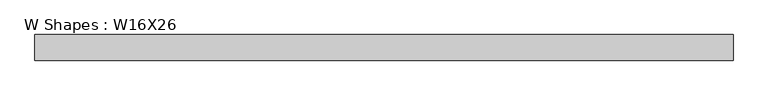
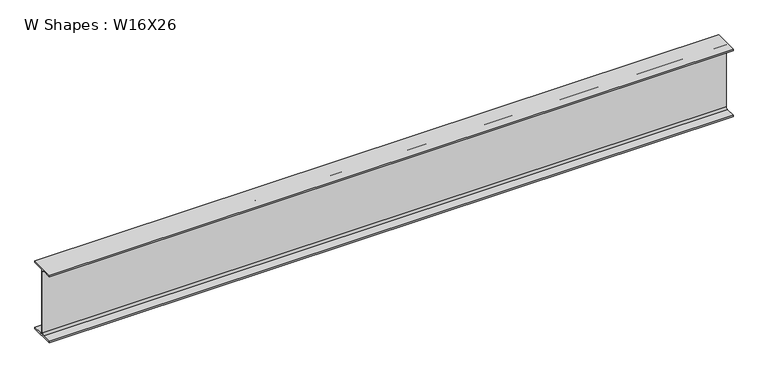
"""IFC4 building model written with IfcOpenShell, lengths in millimetres: beam geometry, W Shapes : W16X26."""

from ifc_helpers import new_model, si_unit, point, frame, frame_2d, origin, place, context, project, spatial, polyline, circle_curve, trimmed, segment, composite_curve, outline, extrude, source, transform, mapped, element, save


def w_shapes_w16x26_2c91abbe(model_context):
    return source(origin(), model_context, "Body", "SweptSolid", [
        extrude(outline(composite_curve([segment(polyline([(69.85, -190.627), (69.85, -199.39), (-69.85, -199.39), (-69.85, -190.627), (-13.3858, -190.627)]), True, "CONTINUOUS"), segment(trimmed(circle_curve(frame_2d((-13.3858, -180.4162)), 10.2108), [point((-13.3858, -190.627))], [point((-3.175, -180.4162))], True, "CARTESIAN"), True, "CONTINUOUS"), segment(polyline([(-3.175, -180.4162), (-3.175, 180.4162)]), True, "CONTINUOUS"), segment(trimmed(circle_curve(frame_2d((-13.3858, 180.4162)), 10.2108), [point((-3.175, 180.4162))], [point((-13.3858, 190.627))], True, "CARTESIAN"), True, "CONTINUOUS"), segment(polyline([(-13.3858, 190.627), (-69.85, 190.627), (-69.85, 199.39), (69.85, 199.39), (69.85, 190.627), (13.3858, 190.627)]), True, "CONTINUOUS"), segment(trimmed(circle_curve(frame_2d((13.3858, 180.4162)), 10.2108), [point((13.3858, 190.627))], [point((3.175, 180.4162))], True, "CARTESIAN"), True, "CONTINUOUS"), segment(polyline([(3.175, 180.4162), (3.175, -180.4162)]), True, "CONTINUOUS"), segment(trimmed(circle_curve(frame_2d((13.3858, -180.4162)), 10.2108), [point((3.175, -180.4162))], [point((13.3858, -190.627))], True, "CARTESIAN"), True, "CONTINUOUS"), segment(polyline([(13.3858, -190.627), (69.85, -190.627)]), True, "CONTINUOUS")], self_intersect=False)), frame((-1905.0, 0.0, 0.0), z_axis=(1.0, 0.0, 0.0), x_axis=(0.0, 1.0, 0.0)), (0.0, 0.0, 1.0), 3810.0),
    ])


if __name__ == "__main__":
    model = new_model("IFC4")
    model_context = context("Model", 3, world=origin())
    ifc_project = project(units=[si_unit("LENGTHUNIT", "METRE", prefix="MILLI")], contexts=[model_context])
    site = spatial("IfcSite", under=ifc_project)
    building = spatial("IfcBuilding", under=site)
    placement = place(None, origin())
    w_shapes_w16x26_shape = w_shapes_w16x26_2c91abbe(model_context)
    element("IfcBeam", 1, ObjectType="W Shapes : W16X26", at=placement, inside=building, context=model_context, shape_type="MappedRepresentation", body=[
        mapped(w_shapes_w16x26_shape, transform((0.0, 0.0, 0.0), x_axis=(1.0, 0.0, 0.0), y_axis=(0.0, 1.0, 0.0), z_axis=(0.0, 0.0, 1.0))),
    ])
    save(model, "model.ifc")

# Revit data of these elements
# Type "W Shapes : W16X26"
#   Section Name Key = "W16x26"
#   Assembly Code = "B10"
#   Width = 5.500"
#   Web Thickness = 0.250"
#   Web Fillet = 0.402"
#   Warping Constant = 565.00 in⁶
#   Torsional Moment of Inertia = 0.262 in⁴
#   Section Area = 7.68 in²
#   Plastic Modulus weak axis = 5.48 in³
#   Plastic Modulus strong axis = 44.20 in³
#   Perimeter = 4.35 ft²/ft
#   Nominal Weight = 26.00 lbf/ft
#   Moment of Inertia weak axis = 9.59 in⁴
#   Moment of Inertia strong axis = 301.00 in⁴
#   Height = 15.700"
#   Flange Thickness = 0.345"
#   Elastic Modulus weak axis = 3.49 in³
#   Elastic Modulus strong axis = 38.40 in³
#   Centroid Vertical = 7.850"
#   Centroid Horizontal = 2.750"
#   Bolt Spacing = 0' - 3 1/2"
#   Length [instance default] = 5' - 0"
#   Structural Material [instance default] = Steel ASTM A992
#   Principal Axes Angle = 0
# Element 1 (IfcBeam, "W Shapes : W16X26")
#   Structural Material = Steel ASTM A36
#   Materials on its faces: "Steel ASTM A36"
# Materials
#   "Steel ASTM A992": class "Metal", colour RGB 199 199 199, transparency 0, Description = "Structural steel 50ksi", Cost = 0
#   "Steel ASTM A36": class "Metal", colour RGB 199 199 199, transparency 0, Description = "Structural steel, ASTM A36 Grade B, mill finish", Cost = 0
